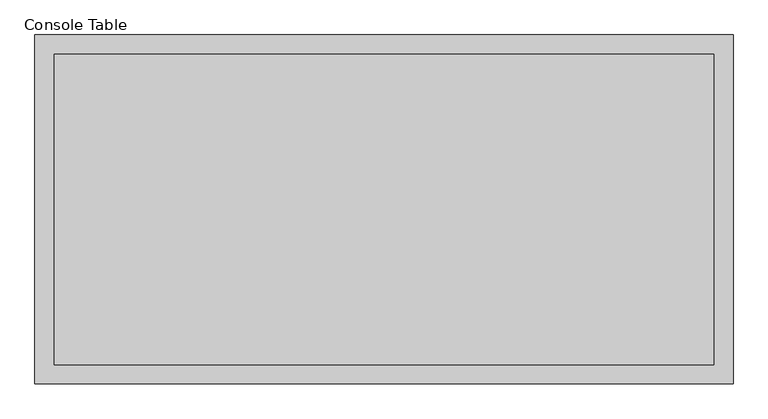
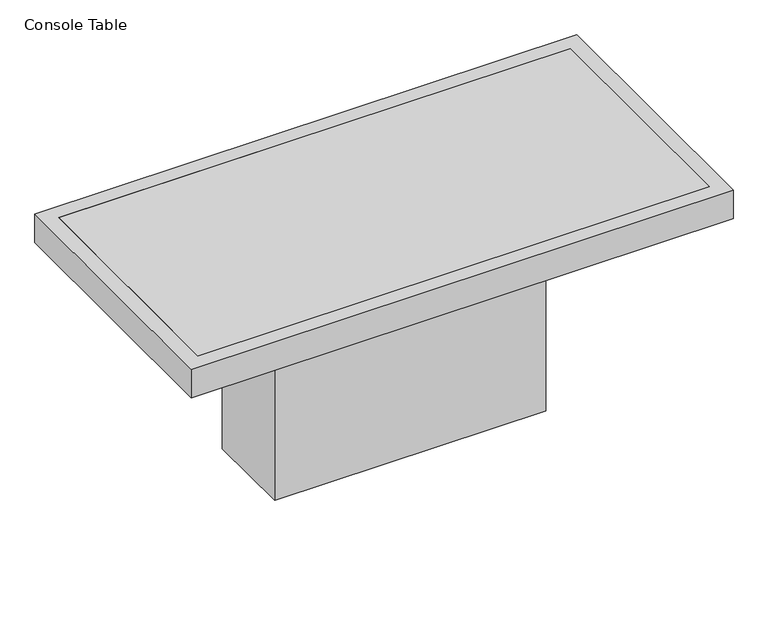
"""IFC4 building model written with IfcOpenShell, lengths in millimetres: furniture geometry, Console Table."""

import ifcopenshell
import ifcopenshell.guid

model = None  # the IFC model being written
_history = None  # IfcOwnerHistory: only IFC2X3 demands one
_inside = {}  # id of a spatial element -> (the spatial element, [elements in it])
_under = {}  # id of a project, library or spatial element -> (it, [spatial elements below it])
_declared = {}  # id of a project -> (the project, [libraries it declares])
_typed = {}  # id of a type object -> (the type object, [elements of that type])
_made_of = {}  # id of a material, layer set ... -> (it, [elements and type objects made of it])


def new_model(schema):
    """Start an empty IFC model of exactly this schema.

    Asked for "IFC4X3", IfcOpenShell would pick the latest addendum, in which some entities
    have other attributes; the version numbers below select the first issue.
    IFC2X3 requires an IfcOwnerHistory on every rooted entity: one is made here for all.
    """
    global model, _history
    if schema == "IFC4X3":
        model = ifcopenshell.file(schema_version=(4, 3, 0, 0))
    else:
        model = ifcopenshell.file(schema=schema)
    _inside.clear()
    _under.clear()
    _declared.clear()
    _typed.clear()
    _made_of.clear()
    _history = None
    if model.schema == "IFC2X3":
        org = make("IfcOrganization", Name="unknown")
        user = make(
            "IfcPersonAndOrganization",
            ThePerson=make("IfcPerson", FamilyName="unknown"),
            TheOrganization=org,
        )
        app = make(
            "IfcApplication",
            ApplicationDeveloper=org,
            Version="unknown",
            ApplicationFullName="unknown",
            ApplicationIdentifier="unknown",
        )
        _history = make(
            "IfcOwnerHistory",
            OwningUser=user,
            OwningApplication=app,
            ChangeAction="ADDED",
            CreationDate=0,
        )
    return model


def make(cls, **values):
    """One entity of the class cls with the attributes given. An attribute that is None is left unset."""
    return model.create_entity(
        cls, **{name: value for name, value in values.items() if value is not None}
    )


def rooted(cls, **values):
    """An entity with a GlobalId (a new one), such as an element, a storey or a relation."""
    return make(cls, GlobalId=ifcopenshell.guid.new(), OwnerHistory=_history, **values)


def si_unit(unit_type, name, prefix=None):
    """IfcSIUnit, for example si_unit("LENGTHUNIT", "METRE", prefix="MILLI")."""
    return make("IfcSIUnit", UnitType=unit_type, Prefix=prefix, Name=name)


def assignment(units):
    """IfcUnitAssignment: the units of a project."""
    return None if units is None else make("IfcUnitAssignment", Units=units)


def point(xyz):
    """IfcCartesianPoint."""
    return None if xyz is None else make("IfcCartesianPoint", Coordinates=xyz)


def direction(xyz):
    """IfcDirection."""
    return None if xyz is None else make("IfcDirection", DirectionRatios=xyz)


def frame(location, z_axis=None, x_axis=None):
    """IfcAxis2Placement3D, a coordinate frame: its origin and axes. An axis left out is left unset."""
    return make(
        "IfcAxis2Placement3D",
        Location=point(location),
        Axis=direction(z_axis),
        RefDirection=direction(x_axis),
    )


def origin():
    """The frame at (0, 0, 0) with its axes left unset."""
    return frame((0.0, 0.0, 0.0))


def origin_with_axes():
    """The frame at (0, 0, 0) with the z axis (0, 0, 1) and the x axis (1, 0, 0) written out."""
    return frame((0.0, 0.0, 0.0), z_axis=(0.0, 0.0, 1.0), x_axis=(1.0, 0.0, 0.0))


def place(relative_to, where):
    """IfcLocalPlacement: puts the frame where relative to a parent placement (None: the world)."""
    return make(
        "IfcLocalPlacement", PlacementRelTo=relative_to, RelativePlacement=where
    )


def context(
    kind, dimensions, precision=None, world=None, true_north=None, identifier=None
):
    """IfcGeometricRepresentationContext, for example the 3D "Model" context."""
    return make(
        "IfcGeometricRepresentationContext",
        ContextIdentifier=identifier,
        ContextType=kind,
        CoordinateSpaceDimension=dimensions,
        Precision=precision,
        WorldCoordinateSystem=world,
        TrueNorth=true_north,
    )


def project(units=None, contexts=None):
    """IfcProject with its units and contexts."""
    return rooted(
        "IfcProject",
        Name="project",
        RepresentationContexts=contexts,
        UnitsInContext=assignment(units),
    )


def spatial(cls, under=None, at=None, **own):
    """A site, building, storey or space (cls), placed at a placement, below another one or the project."""
    s = rooted(cls, ObjectPlacement=at, **own)
    if under is not None:
        _under.setdefault(under.id(), (under, []))[1].append(s)
    return s


def polyline(points):
    """IfcPolyline through the points."""
    return make("IfcPolyline", Points=[point(p) for p in points])


def outline(outer, holes=None, kind="AREA"):
    """IfcArbitraryClosedProfileDef: a profile drawn as a closed curve; with holes, ...WithVoids."""
    if holes is None:
        return make("IfcArbitraryClosedProfileDef", ProfileType=kind, OuterCurve=outer)
    return make(
        "IfcArbitraryProfileDefWithVoids",
        ProfileType=kind,
        OuterCurve=outer,
        InnerCurves=holes,
    )


def extrude(swept, where, along, depth):
    """IfcExtrudedAreaSolid: the profile swept, set in the frame where, extruded along a direction by depth."""
    return make(
        "IfcExtrudedAreaSolid",
        SweptArea=swept,
        Position=where,
        ExtrudedDirection=direction(along),
        Depth=depth,
    )


def shape(context_of_items, identifier, shape_type, items):
    """IfcShapeRepresentation: the items that make up one representation, for example the "Body"."""
    return make(
        "IfcShapeRepresentation",
        ContextOfItems=context_of_items,
        RepresentationIdentifier=identifier,
        RepresentationType=shape_type,
        Items=items,
    )


def source(mapping_origin, context_of_items, identifier, shape_type, items):
    """IfcRepresentationMap: a shape defined once, which mapped items show again and again."""
    return make(
        "IfcRepresentationMap",
        MappingOrigin=mapping_origin,
        MappedRepresentation=shape(context_of_items, identifier, shape_type, items),
    )


def transform(
    local_origin,
    x_axis=None,
    y_axis=None,
    z_axis=None,
    scale=None,
    scale2=None,
    scale3=None,
    uniform=True,
):
    """IfcCartesianTransformationOperator3D, or its non-uniform kind. x_axis, y_axis, z_axis: its Axis1, 2, 3."""
    if uniform:
        return make(
            "IfcCartesianTransformationOperator3D",
            Axis1=direction(x_axis),
            Axis2=direction(y_axis),
            LocalOrigin=point(local_origin),
            Scale=scale,
            Axis3=direction(z_axis),
        )
    return make(
        "IfcCartesianTransformationOperator3DnonUniform",
        Axis1=direction(x_axis),
        Axis2=direction(y_axis),
        LocalOrigin=point(local_origin),
        Scale=scale,
        Axis3=direction(z_axis),
        Scale2=scale2,
        Scale3=scale3,
    )


def mapped(mapping_source, mapping_target):
    """IfcMappedItem: shows the shape of a source again, moved by a transform."""
    return make(
        "IfcMappedItem", MappingSource=mapping_source, MappingTarget=mapping_target
    )


def made_of(thing, what):
    """Note that an element or type object is made of a material, layer set ...; save() writes the relation."""
    if what is not None:
        _made_of.setdefault(what.id(), (what, []))[1].append(thing)
    return thing


def element(
    cls,
    number,
    at=None,
    inside=None,
    cuts=None,
    type_object=None,
    material=None,
    context=None,
    identifier="Body",
    shape_type=None,
    held_by="IfcProductDefinitionShape",
    body=None,
    shapes=None,
    **own,
):
    """One element of the class cls, such as IfcWall. Its Tag is "e" and its number.

    at: its placement. inside: the storey or other place that contains it. cuts: it is an
    opening in that element (IfcRelVoidsElement). A single representation is given by context,
    identifier, shape_type and body (its items); several are given by shapes. held_by: the class
    of the entity that holds the representations. save() writes the other relations.
    """
    e = rooted(cls, Tag="e%d" % number, ObjectPlacement=at, **own)
    if body is not None:
        shapes = [shape(context, identifier, shape_type, body)]
    if shapes is not None:
        e.Representation = make(held_by, Representations=shapes)
    if inside is not None:
        _inside.setdefault(inside.id(), (inside, []))[1].append(e)
    if cuts is not None:
        rooted(
            "IfcRelVoidsElement", RelatingBuildingElement=cuts, RelatedOpeningElement=e
        )
    if type_object is not None:
        _typed.setdefault(type_object.id(), (type_object, []))[1].append(e)
    return made_of(e, material)


def aggregate(whole, parts):
    """IfcRelAggregates: a whole, such as a stair, and the parts it consists of."""
    return rooted("IfcRelAggregates", RelatingObject=whole, RelatedObjects=parts)


def save(model, path):
    """Write the relations noted so far, then the file.

    IfcRelAggregates (storeys below a building ...), IfcRelContainedInSpatialStructure (elements
    in a storey), IfcRelDefinesByType, IfcRelAssociatesMaterial and IfcRelDeclares: one each for
    every whole, place, type object, material and project.
    """
    for whole, parts in _under.values():
        aggregate(whole, parts)
    for where, things in _inside.values():
        rooted(
            "IfcRelContainedInSpatialStructure",
            RelatedElements=things,
            RelatingStructure=where,
        )
    for kind, things in _typed.values():
        rooted("IfcRelDefinesByType", RelatedObjects=things, RelatingType=kind)
    for what, things in _made_of.values():
        rooted("IfcRelAssociatesMaterial", RelatedObjects=things, RelatingMaterial=what)
    for by, libraries in _declared.values():
        rooted("IfcRelDeclares", RelatingContext=by, RelatedDefinitions=libraries)
    model.write(path)


def console_table_526d3b16(model_context):
    return source(origin(), model_context, "Body", "SweptSolid", [
        extrude(outline(polyline([(457.2, 152.4), (457.2, -152.4), (-457.2, -152.4), (-457.2, 152.4), (457.2, 152.4)])), origin_with_axes(), (0.0, 0.0, 1.0), 787.4),
        extrude(outline(polyline([(-863.6, -406.4), (-863.6, 406.4), (863.6, 406.4), (863.6, -406.4), (-863.6, -406.4)])), frame((0.0, 0.0, 787.4), z_axis=(0.0, 0.0, 1.0), x_axis=(1.0, 0.0, 0.0)), (0.0, 0.0, 1.0), 25.4),
        extrude(outline(polyline([(914.4, 457.2), (914.4, -457.2), (-914.4, -457.2), (-914.4, 457.2), (914.4, 457.2)]), holes=[polyline([(863.6, 406.4), (-863.6, 406.4), (-863.6, -406.4), (863.6, -406.4), (863.6, 406.4)])]), frame((0.0, 0.0, 711.2), z_axis=(0.0, 0.0, 1.0), x_axis=(1.0, 0.0, 0.0)), (0.0, 0.0, 1.0), 101.6),
    ])


if __name__ == "__main__":
    model = new_model("IFC4")
    model_context = context("Model", 3, world=origin())
    ifc_project = project(units=[si_unit("LENGTHUNIT", "METRE", prefix="MILLI")], contexts=[model_context])
    site = spatial("IfcSite", under=ifc_project)
    building = spatial("IfcBuilding", under=site)
    placement = place(None, origin())
    console_table_shape = console_table_526d3b16(model_context)
    element("IfcFurniture", 1, ObjectType="Console Table : 72\" L  x 36\" W x 32\" H", at=placement, inside=building, context=model_context, shape_type="MappedRepresentation", body=[
        mapped(console_table_shape, transform((0.0, 0.0, 0.0), x_axis=(1.0, 0.0, 0.0), y_axis=(0.0, 1.0, 0.0), z_axis=(0.0, 0.0, 1.0))),
    ])
    save(model, "model.ifc")

# Revit data of these elements
# Project information
#   SR Document GUID = "e87cf156-1ea9-4512-a4ef-a5481400b45a"
# Type "Console Table : 72\" L  x 36\" W x 32\" H"
#   Table Width = 3' - 0"
#   Table Length = 6' - 0"
#   Table Height = 2' - 8"
#   Pedestal Width = 1' - 0"
#   Pedestal Length = 3' - 0"
#   Frame Thickness = 0' - 2"
#   Frame Height = 0' - 4"
#   Table Surface [instance default] = none
#   Table Frame [instance default] = none
#   Pedestal [instance default] = none
#   Default Elevation = 0
#   Assembly Code = ""
